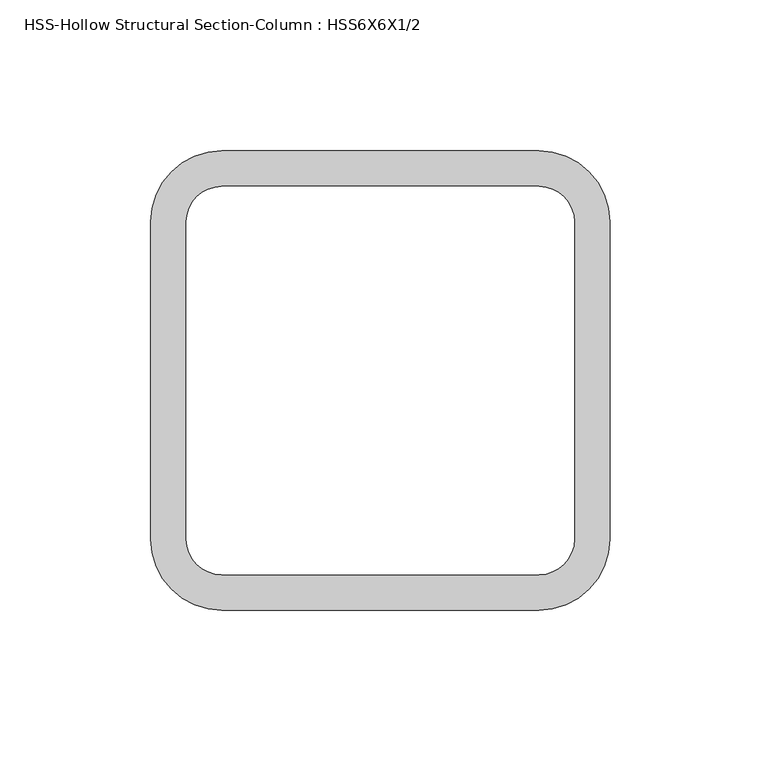
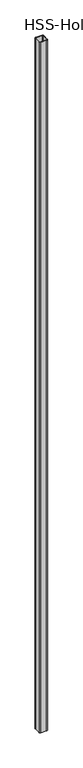
"""IFC4 building model written with IfcOpenShell, lengths in millimetres: column geometry, HSS-Hollow Structural Section-Column : HSS6X6X1/2."""

from ifc_helpers import new_model, si_unit, point, frame, frame_2d, origin, place, context, project, spatial, polyline, circle_curve, trimmed, segment, composite_curve, outline, extrude, source, transform, mapped, element, save


def hss_hollow_structural_section_column_hss6x6x1_2_b8c6504c(model_context):
    return source(origin(), model_context, "Body", "SweptSolid", [
        extrude(outline(composite_curve([segment(trimmed(circle_curve(frame_2d((52.578, 52.578)), 23.622), [point((52.578, 76.2))], [point((76.2, 52.578))], False, "CARTESIAN"), True, "CONTINUOUS"), segment(polyline([(76.2, 52.578), (76.2, -52.578)]), True, "CONTINUOUS"), segment(trimmed(circle_curve(frame_2d((52.578, -52.578)), 23.622), [point((76.2, -52.578))], [point((52.578, -76.2))], False, "CARTESIAN"), True, "CONTINUOUS"), segment(polyline([(52.578, -76.2), (-52.578, -76.2)]), True, "CONTINUOUS"), segment(trimmed(circle_curve(frame_2d((-52.578, -52.578)), 23.622), [point((-52.578, -76.2))], [point((-76.2, -52.578))], False, "CARTESIAN"), True, "CONTINUOUS"), segment(polyline([(-76.2, -52.578), (-76.2, 52.578)]), True, "CONTINUOUS"), segment(trimmed(circle_curve(frame_2d((-52.578, 52.578)), 23.622), [point((-76.2, 52.578))], [point((-52.578, 76.2))], False, "CARTESIAN"), True, "CONTINUOUS"), segment(polyline([(-52.578, 76.2), (52.578, 76.2)]), True, "CONTINUOUS")], self_intersect=False), holes=[composite_curve([segment(polyline([(52.578, 64.389), (-52.578, 64.389)]), True, "CONTINUOUS"), segment(trimmed(circle_curve(frame_2d((-52.578, 52.578)), 11.811), [point((-52.578, 64.389))], [point((-64.389, 52.578))], True, "CARTESIAN"), True, "CONTINUOUS"), segment(polyline([(-64.389, 52.578), (-64.389, -52.578)]), True, "CONTINUOUS"), segment(trimmed(circle_curve(frame_2d((-52.578, -52.578)), 11.811), [point((-64.389, -52.578))], [point((-52.578, -64.389))], True, "CARTESIAN"), True, "CONTINUOUS"), segment(polyline([(-52.578, -64.389), (52.578, -64.389)]), True, "CONTINUOUS"), segment(trimmed(circle_curve(frame_2d((52.578, -52.578)), 11.811), [point((52.578, -64.389))], [point((64.389, -52.578))], True, "CARTESIAN"), True, "CONTINUOUS"), segment(polyline([(64.389, -52.578), (64.389, 52.578)]), True, "CONTINUOUS"), segment(trimmed(circle_curve(frame_2d((52.578, 52.578)), 11.811), [point((64.389, 52.578))], [point((52.578, 64.389))], True, "CARTESIAN"), True, "CONTINUOUS")], self_intersect=False)]), frame((0.0, 0.0, -609.6), z_axis=(0.0, 0.0, 1.0), x_axis=(1.0, 0.0, 0.0)), (0.0, 0.0, 1.0), 13157.2),
    ])


if __name__ == "__main__":
    model = new_model("IFC4")
    model_context = context("Model", 3, world=origin())
    ifc_project = project(units=[si_unit("LENGTHUNIT", "METRE", prefix="MILLI")], contexts=[model_context])
    site = spatial("IfcSite", under=ifc_project)
    building = spatial("IfcBuilding", under=site)
    placement = place(None, origin())
    hss_hollow_structural_section_column_hss6x6x1_2_shape = hss_hollow_structural_section_column_hss6x6x1_2_b8c6504c(model_context)
    element("IfcColumn", 1, ObjectType="HSS-Hollow Structural Section-Column : HSS6X6X1/2", at=placement, inside=building, context=model_context, shape_type="MappedRepresentation", body=[
        mapped(hss_hollow_structural_section_column_hss6x6x1_2_shape, transform((0.0, 0.0, 0.0), x_axis=(1.0, 0.0, 0.0), y_axis=(0.0, 1.0, 0.0), z_axis=(0.0, 0.0, 1.0))),
    ])
    save(model, "model.ifc")

# Revit data of these elements
# Type "HSS-Hollow Structural Section-Column : HSS6X6X1/2"
#   Assembly Code = "B10"
#   Shape = "Square"
#   W = 35.1
#   Ht = 0' - 6"
#   b = 0' - 6"
#   kr = 0' - 0.93"
#   t = 0' - 0.465"
#   A = 0.0676389 SF
#   Structural Material [instance default] = Steel ASTM A500, Grade B, Rectangular and Square
# Element 1 (IfcColumn, "HSS-Hollow Structural Section-Column : HSS6X6X1/2")
#   Materials on its faces: "Steel ASTM A500, Grade B, Rectangular and Square"
# Materials
#   "Steel ASTM A500, Grade B, Rectangular and Square": class "Metal", colour RGB 199 199 199, transparency 0, Description = "Carbon steel", Cost = 0
